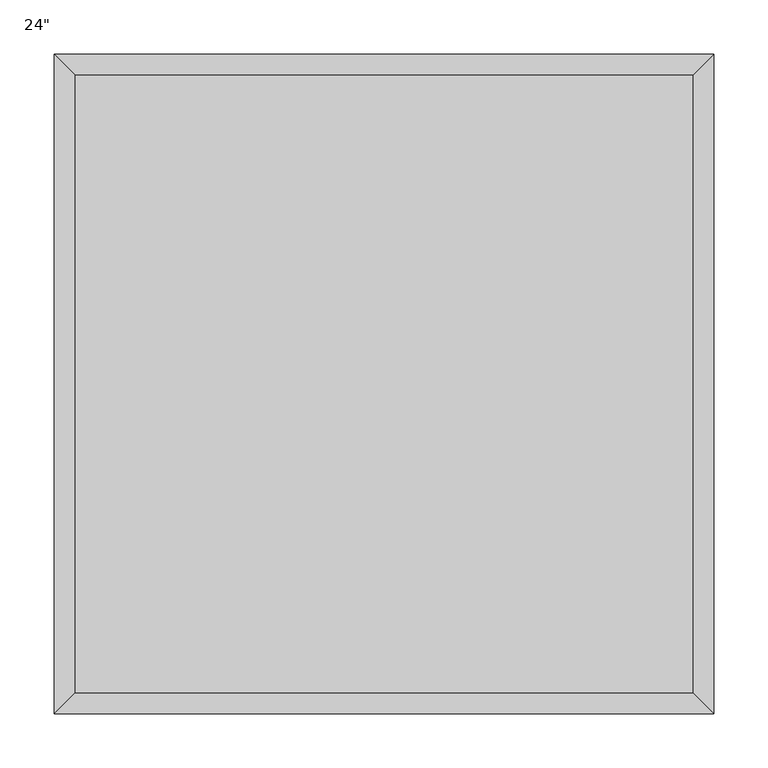
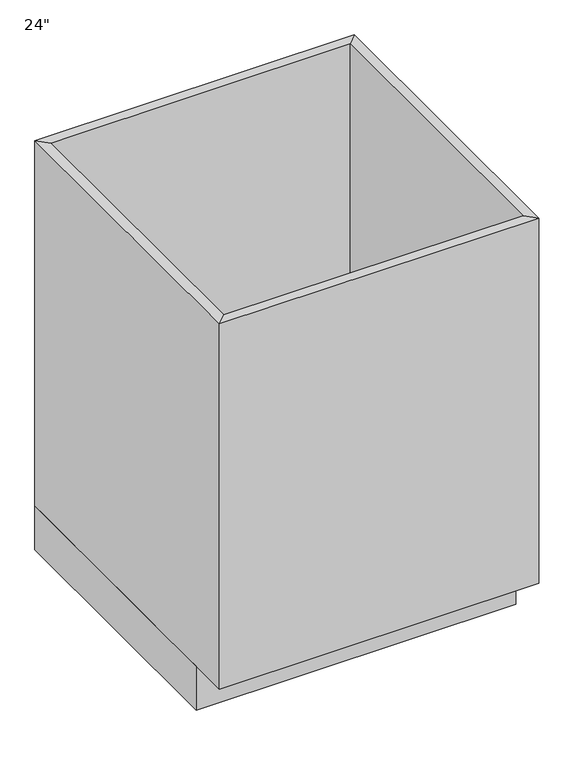
"""IFC4 building model written with IfcOpenShell, lengths in millimetres: furniture geometry."""

from ifc_helpers import new_model, si_unit, frame, origin, origin_with_axes, place, context, project, spatial, polyline, outline, extrude, faceted_brep, source, transform, mapped, element, save


def furniture_31151d79(model_context):
    return source(origin(), model_context, "Body", "SolidModel", [
        extrude(outline(polyline([(304.4877049, -19.05), (304.4877049, -590.55), (-267.0122951, -590.55), (-267.0122951, -19.05), (304.4877049, -19.05)])), frame((0.0, 0.0, 88.9), z_axis=(0.0, 0.0, 1.0), x_axis=(1.0, 0.0, 0.0)), (0.0, 0.0, 1.0), 19.05),
        faceted_brep([(304.4877049, -590.55, 825.5), (304.4877049, -590.55, 88.9), (-267.0122951, -590.55, 88.9), (-267.0122951, -590.55, 825.5), (323.5377049, -609.6, 825.5), (-286.0622951, -609.6, 825.5), (323.5377049, -609.6, 88.9), (-286.0622951, -609.6, 88.9), (-267.0122951, -19.05, 88.9), (-267.0122951, -19.05, 825.5), (-286.0622951, 0.0, 825.5), (-286.0622951, 0.0, 88.9), (304.4877049, -19.05, 88.9), (304.4877049, -19.05, 825.5), (323.5377049, 0.0, 825.5), (323.5377049, 0.0, 88.9)], [[[0, 1, 2, 3]], [[4, 0, 3, 5]], [[6, 4, 5, 7]], [[1, 6, 7, 2]], [[3, 2, 8, 9]], [[5, 3, 9, 10]], [[7, 5, 10, 11]], [[2, 7, 11, 8]], [[9, 8, 12, 13]], [[10, 9, 13, 14]], [[11, 10, 14, 15]], [[8, 11, 15, 12]], [[13, 12, 1, 0]], [[14, 13, 0, 4]], [[15, 14, 4, 6]], [[12, 15, 6, 1]]]),
        extrude(outline(polyline([(323.5377049, 0.0), (323.5377049, -533.4), (-286.0622951, -533.4), (-286.0622951, 0.0), (323.5377049, 0.0)])), origin_with_axes(), (0.0, 0.0, 1.0), 88.9),
    ])


if __name__ == "__main__":
    model = new_model("IFC4")
    model_context = context("Model", 3, world=origin())
    ifc_project = project(units=[si_unit("LENGTHUNIT", "METRE", prefix="MILLI")], contexts=[model_context])
    site = spatial("IfcSite", under=ifc_project)
    building = spatial("IfcBuilding", under=site)
    placement = place(None, origin())
    furniture_shape = furniture_31151d79(model_context)
    element("IfcFurniture", 1, ObjectType="Base Cabinet-Single Door & Drawer : 24\"", at=placement, inside=building, context=model_context, shape_type="MappedRepresentation", body=[
        mapped(furniture_shape, transform((0.0, 0.0, 0.0), x_axis=(1.0, 0.0, 0.0), y_axis=(0.0, 1.0, 0.0), z_axis=(0.0, 0.0, 1.0))),
    ])
    save(model, "model.ifc")

# Revit data of these elements
# Type "Base Cabinet-Single Door & Drawer : 24\""
#   Depth = 2' - 0"
#   Height = 2' - 8 1/2"
#   Toe Depth = 0' - 3"
#   Toe Height = 0' - 3 1/2"
#   Width = 2' - 0"
# Element 1 (IfcFurniture, "Base Cabinet-Single Door & Drawer : 24\"")
#   Materials on its faces: "CASEWORK"
# Materials
#   "CASEWORK": class "Generic", colour RGB 181 181 181, transparency 0, Cost = 0
